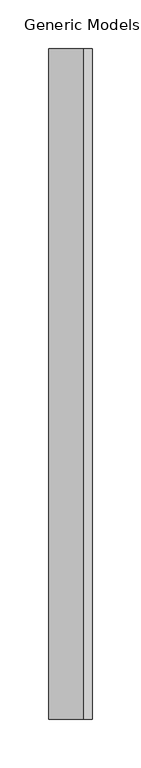
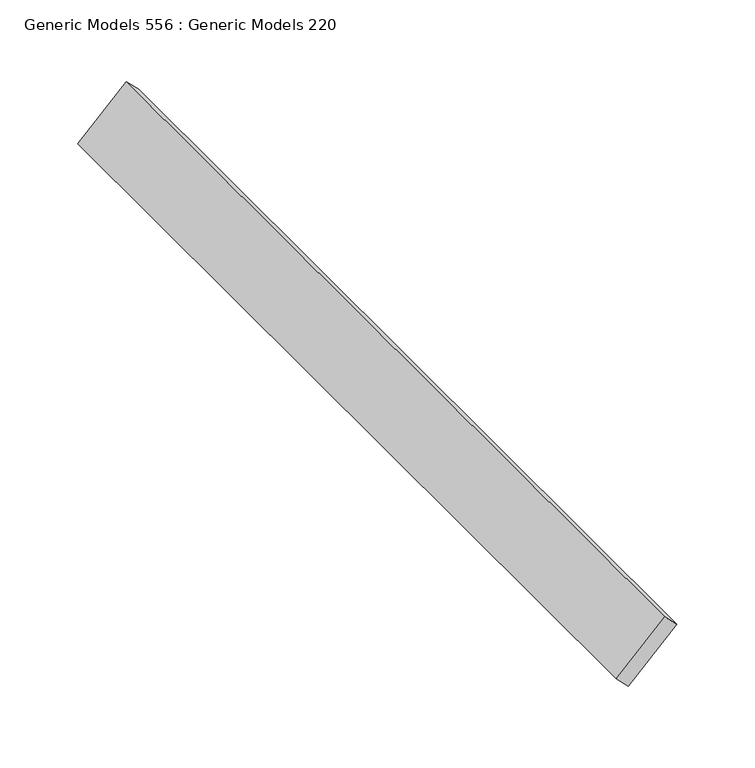
"""IFC4 building model written with IfcOpenShell, lengths in millimetres: proxy geometry, Generic Models 556 : Generic Models 220."""

from ifc_helpers import new_model, si_unit, frame, origin, place, context, project, spatial, polyline, outline, extrude, source, transform, mapped, element, save


def generic_models_556_generic_models_220_bf90978c(model_context):
    return source(origin(), model_context, "Body", "SweptSolid", [
        extrude(outline(polyline([(0.0, -12.7000001), (0.0, 0.0), (690.8142348, 0.0), (690.8142348, -12.7000001), (0.0, -12.7000001)])), frame((7841.3059863, 4539.4872686, 124493.6399101), z_axis=(0.7071067811868034, 0.0, 0.7071067811862918), x_axis=(0.0, -1.0, 0.0)), (0.0, 0.0, 1.0), 50.8),
    ])


if __name__ == "__main__":
    model = new_model("IFC4")
    model_context = context("Model", 3, world=origin())
    ifc_project = project(units=[si_unit("LENGTHUNIT", "METRE", prefix="MILLI")], contexts=[model_context])
    site = spatial("IfcSite", under=ifc_project)
    building = spatial("IfcBuilding", under=site)
    placement = place(None, origin())
    generic_models_556_generic_models_220_shape = generic_models_556_generic_models_220_bf90978c(model_context)
    element("IfcBuildingElementProxy", 1, Name="Generic Models 556 : Generic Models 220", ObjectType="Generic Models 556 : Generic Models 220", at=placement, inside=building, context=model_context, shape_type="MappedRepresentation", body=[
        mapped(generic_models_556_generic_models_220_shape, transform((0.0, 0.0, 0.0), x_axis=(1.0, 0.0, 0.0), y_axis=(0.0, 1.0, 0.0), z_axis=(0.0, 0.0, 1.0))),
    ])
    save(model, "model.ifc")

# Revit data of these elements
# Element 1 (IfcBuildingElementProxy, "Generic Models 556 : Generic Models 220")
#   Materials on its faces: "_WOOD TONE ALUMINUM EXTRUSION SLAT BY KNOTWOOD"
# Materials
#   "_WOOD TONE ALUMINUM EXTRUSION SLAT BY KNOTWOOD": class "Generic", colour RGB 177 130 114, transparency 0, Cost = 0
